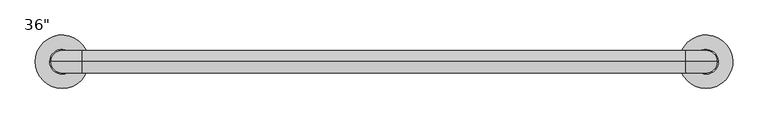
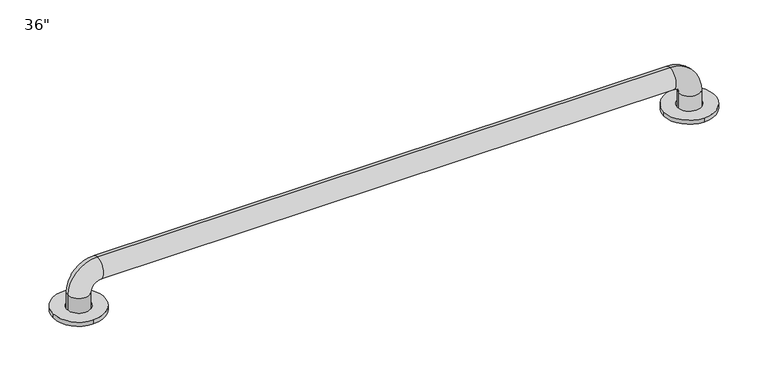
"""IFC4 building model written with IfcOpenShell, lengths in millimetres: proxy geometry."""

from ifc_helpers import new_model, si_unit, point, frame, frame_2d, origin, origin_with_axes, origin_2d, place, context, project, spatial, circle_curve, ellipse_curve, trimmed, segment, composite_curve, outline, extrude, source, transform, mapped, element, save
from ifc_brep_helpers import plane_surface, cylinder_surface, revolved_surface, advanced_brep


def proxy_70f9e0ae(model_context):
    return source(origin(), model_context, "Body", "SolidModel", [
        extrude(outline(composite_curve([segment(trimmed(circle_curve(frame_2d((914.4, 0.0)), 38.1), [point((876.3, 0.0))], [point((914.4, -38.1))], False, "CARTESIAN"), True, "CONTINUOUS"), segment(trimmed(circle_curve(frame_2d((914.4, 0.0)), 38.1), [point((914.4, -38.1))], [point((876.3, 0.0))], False, "CARTESIAN"), True, "CONTINUOUS")], self_intersect=False), holes=[composite_curve([segment(trimmed(circle_curve(frame_2d((914.4, 0.0)), 17.4625), [point((896.9375, 0.0))], [point((914.4, -17.4625))], True, "CARTESIAN"), True, "CONTINUOUS"), segment(trimmed(circle_curve(frame_2d((914.4, 0.0)), 17.4625), [point((914.4, -17.4625))], [point((896.9375, 0.0))], True, "CARTESIAN"), True, "CONTINUOUS")], self_intersect=False)]), origin_with_axes(), (0.0, 0.0, 1.0), 6.35),
        extrude(outline(composite_curve([segment(trimmed(circle_curve(origin_2d(), 38.1), [point((-38.1, 0.0))], [point((0.0, -38.1))], False, "CARTESIAN"), True, "CONTINUOUS"), segment(trimmed(circle_curve(origin_2d(), 38.1), [point((0.0, -38.1))], [point((-38.1, 0.0))], False, "CARTESIAN"), True, "CONTINUOUS")], self_intersect=False), holes=[composite_curve([segment(trimmed(circle_curve(origin_2d(), 17.4625), [point((-17.4625, 0.0))], [point((0.0, -17.4625))], True, "CARTESIAN"), True, "CONTINUOUS"), segment(trimmed(circle_curve(origin_2d(), 17.4625), [point((0.0, -17.4625))], [point((-17.4625, 0.0))], True, "CARTESIAN"), True, "CONTINUOUS")], self_intersect=False)]), origin_with_axes(), (0.0, 0.0, 1.0), 6.35),
        advanced_brep(
        [(930.275, 0.0, 0.0), (898.525, 0.0, 0.0), (930.275, 0.0, 28.575), (898.525, 0.0, 28.575), (885.825, 0.0, 41.275), (885.825, 0.0, 73.025), (28.575, 0.0, 73.025), (28.575, 0.0, 41.275), (15.875, 0.0, 28.575), (-15.875, 0.0, 28.575), (-15.875, 0.0, 0.0), (15.875, 0.0, 0.0)],
        [
            (0, 1, circle_curve(frame((914.4, 0.0, 0.0), z_axis=(0.0, 0.0, -1.0), x_axis=(-1.0, 0.0, 0.0)), 15.875)),
            (1, 0, circle_curve(frame((914.4, 0.0, 0.0), z_axis=(0.0, 0.0, -1.0), x_axis=(-1.0, 0.0, 0.0)), 15.875)),
            (0, 2),
            (2, 3, circle_curve(frame((914.4, 0.0, 28.575), z_axis=(0.0, 0.0, -1.0), x_axis=(-1.0, 0.0, 0.0)), 15.875)),
            (3, 1),
            (3, 2, circle_curve(frame((914.4, 0.0, 28.575), z_axis=(0.0, 0.0, -1.0), x_axis=(-1.0, 0.0, 0.0)), 15.875)),
            (4, 3, circle_curve(frame((885.825, 0.0, 28.575), z_axis=(0.0, 1.0, 0.0), x_axis=(1.0, 0.0, 0.0)), 12.7)),
            (2, 5, circle_curve(frame((885.825, 0.0, 28.575), z_axis=(0.0, -1.0, 0.0), x_axis=(1.0, 0.0, 0.0)), 44.45)),
            (5, 4, circle_curve(frame((885.825, 0.0, 57.15), z_axis=(1.0, 0.0, 0.0), x_axis=(0.0, 0.0, -1.0)), 15.875)),
            (4, 5, circle_curve(frame((885.825, 0.0, 57.15), z_axis=(1.0, 0.0, 0.0), x_axis=(0.0, 0.0, -1.0)), 15.875)),
            (5, 6),
            (6, 7, circle_curve(frame((28.575, 0.0, 57.15), z_axis=(1.0, 0.0, 0.0), x_axis=(0.0, 0.0, -1.0)), 15.875)),
            (7, 4),
            (7, 6, circle_curve(frame((28.575, 0.0, 57.15), z_axis=(1.0, 0.0, 0.0), x_axis=(0.0, 0.0, -1.0)), 15.875)),
            (8, 7, circle_curve(frame((28.575, 0.0, 28.575), z_axis=(0.0, 1.0, 0.0), x_axis=(0.0, 0.0, 1.0)), 12.7)),
            (6, 9, circle_curve(frame((28.575, 0.0, 28.575), z_axis=(0.0, -1.0, 0.0), x_axis=(0.0, 0.0, 1.0)), 44.45)),
            (9, 8, circle_curve(frame((0.0, 0.0, 28.575), z_axis=(0.0, 0.0, 1.0), x_axis=(1.0, 0.0, 0.0)), 15.875)),
            (8, 9, circle_curve(frame((0.0, 0.0, 28.575), z_axis=(0.0, 0.0, 1.0), x_axis=(1.0, 0.0, 0.0)), 15.875)),
            (10, 11, circle_curve(frame((0.0, 0.0, 0.0), z_axis=(0.0, 0.0, -1.0), x_axis=(1.0, 0.0, 0.0)), 15.875)),
            (11, 10, circle_curve(frame((0.0, 0.0, 0.0), z_axis=(0.0, 0.0, -1.0), x_axis=(1.0, 0.0, 0.0)), 15.875)),
            (9, 10),
            (11, 8),
        ],
        [
            plane_surface(frame((914.4, 0.0, 0.0), z_axis=(0.0, 0.0, -1.0), x_axis=(0.0, -1.0, 0.0))),
            cylinder_surface(frame((914.4, 0.0, 0.0), z_axis=(0.0, 0.0, -1.0), x_axis=(-1.0, 0.0, 0.0)), 15.875),
            revolved_surface(trimmed(ellipse_curve(frame((914.4, 0.0, 28.575), z_axis=(0.0, 0.0, -1.0), x_axis=(-1.0, 0.0, 0.0)), 15.875, 15.875), [point((930.275, 0.0, 28.575))], [point((898.525, 0.0, 28.575))], True, "CARTESIAN"), (885.825, 0.0, 28.575), (0.0, -1.0, 0.0)),
            revolved_surface(trimmed(ellipse_curve(frame((914.4, 0.0, 28.575), z_axis=(0.0, 0.0, -1.0), x_axis=(-1.0, 0.0, 0.0)), 15.875, 15.875), [point((898.525, 0.0, 28.575))], [point((930.275, 0.0, 28.575))], True, "CARTESIAN"), (885.825, 0.0, 28.575), (0.0, -1.0, 0.0)),
            cylinder_surface(frame((885.825, 0.0, 57.15), z_axis=(1.0, 0.0, 0.0), x_axis=(0.0, 0.0, -1.0)), 15.875),
            revolved_surface(trimmed(ellipse_curve(frame((28.575, 0.0, 57.15), z_axis=(1.0, 0.0, 0.0), x_axis=(0.0, 0.0, -1.0)), 15.875, 15.875), [point((28.575, 0.0, 73.025))], [point((28.575, 0.0, 41.275))], True, "CARTESIAN"), (28.575, 0.0, 28.575), (0.0, -1.0, 0.0)),
            revolved_surface(trimmed(ellipse_curve(frame((28.575, 0.0, 57.15), z_axis=(1.0, 0.0, 0.0), x_axis=(0.0, 0.0, -1.0)), 15.875, 15.875), [point((28.575, 0.0, 41.275))], [point((28.575, 0.0, 73.025))], True, "CARTESIAN"), (28.575, 0.0, 28.575), (0.0, -1.0, 0.0)),
            plane_surface(frame((0.0, 0.0, 0.0), z_axis=(0.0, 0.0, -1.0), x_axis=(0.0, -1.0, 0.0))),
            cylinder_surface(frame((0.0, 0.0, 28.575), z_axis=(0.0, 0.0, 1.0), x_axis=(1.0, 0.0, 0.0)), 15.875),
        ],
        [
            (0, [[1, 2]]),
            (1, [[-1, 3, 4, 5]]),
            (1, [[-2, -5, 6, -3]]),
            (2, [[7, -4, 8, 9]]),
            (3, [[-8, -6, -7, 10]]),
            (4, [[-9, 11, 12, 13]]),
            (4, [[-10, -13, 14, -11]]),
            (5, [[15, -12, 16, 17]]),
            (6, [[-16, -14, -15, 18]]),
            (7, [[19, 20]]),
            (8, [[-17, 21, -20, 22]]),
            (8, [[-18, -22, -19, -21]]),
        ],
    ),
    ])


if __name__ == "__main__":
    model = new_model("IFC4")
    model_context = context("Model", 3, world=origin())
    ifc_project = project(units=[si_unit("LENGTHUNIT", "METRE", prefix="MILLI")], contexts=[model_context])
    site = spatial("IfcSite", under=ifc_project)
    building = spatial("IfcBuilding", under=site)
    placement = place(None, origin())
    proxy_shape = proxy_70f9e0ae(model_context)
    element("IfcBuildingElementProxy", 1, Name="Seqm-Grab Bar : 36\"", ObjectType="Seqm-Grab Bar : 36\"", at=placement, inside=building, context=model_context, shape_type="MappedRepresentation", body=[
        mapped(proxy_shape, transform((0.0, 0.0, 0.0), x_axis=(1.0, 0.0, 0.0), y_axis=(0.0, 1.0, 0.0), z_axis=(0.0, 0.0, 1.0))),
    ])
    save(model, "model.ifc")

# Revit data of these elements
# Type "Seqm-Grab Bar : 36\""
#   Spec Number = "10 28 00"
#   Spec Description = "36\" GRAB BAR"
#   Length = 3' - 0"
#   Default Elevation = 4' - 0"
#   Grab Bar Material = GRAB BARS - AT ADA RESTROOMS ONLY
# Element 1 (IfcBuildingElementProxy, "Seqm-Grab Bar : 36\"")
#   Materials on its faces: "GRAB BARS - AT ADA RESTROOMS ONLY"
# Materials
#   "GRAB BARS - AT ADA RESTROOMS ONLY": class "Generic", colour RGB 120 120 120, transparency 0, Cost = 0
